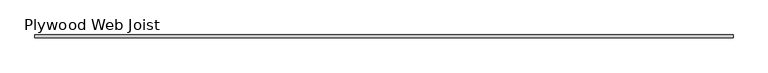
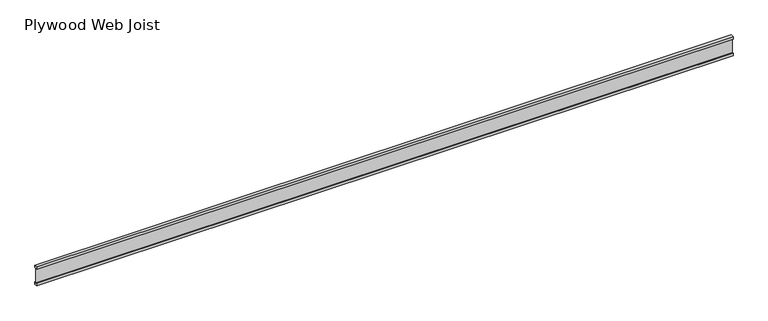
"""IFC4 building model written with IfcOpenShell, lengths in millimetres: beam geometry, Plywood Web Joist : TJI (T.B.D.)."""

from ifc_helpers import new_model, si_unit, frame, origin, place, context, project, spatial, polyline, outline, extrude, source, transform, mapped, element, save


def plywood_web_joist_03ebe8c7(model_context):
    return source(origin(), model_context, "Body", "SweptSolid", [
        extrude(outline(polyline([(-22.225, 150.8125), (22.225, 150.8125), (22.225, 112.7125), (4.7625, 112.7125), (4.7625, 119.0625), (-4.7625, 119.0625), (-4.7625, 112.7125), (-22.225, 112.7125), (-22.225, 150.8125)])), frame((-5185.9151287, 0.0, 0.0), z_axis=(1.0, 0.0, 0.0), x_axis=(0.0, 1.0, 0.0)), (0.0, 0.0, 1.0), 10371.8302575),
        extrude(outline(polyline([(22.225, -112.7125), (22.225, -150.8125), (-22.225, -150.8125), (-22.225, -112.7125), (-4.7625, -112.7125), (-4.7625, -118.3285374), (4.7625, -118.3285374), (4.7625, -112.7125), (22.225, -112.7125)])), frame((-5185.9151287, 0.0, 0.0), z_axis=(1.0, 0.0, 0.0), x_axis=(0.0, 1.0, 0.0)), (0.0, 0.0, 1.0), 10371.8302575),
        extrude(outline(polyline([(5185.9151287, 4.7625), (5185.9151287, -4.7625), (-5185.9151287, -4.7625), (-5185.9151287, 4.7625), (5185.9151287, 4.7625)])), frame((0.0, 0.0, -118.3285374), z_axis=(0.0, 0.0, 1.0), x_axis=(1.0, 0.0, 0.0)), (0.0, 0.0, 1.0), 237.3910374),
    ])


if __name__ == "__main__":
    model = new_model("IFC4")
    model_context = context("Model", 3, world=origin())
    ifc_project = project(units=[si_unit("LENGTHUNIT", "METRE", prefix="MILLI")], contexts=[model_context])
    site = spatial("IfcSite", under=ifc_project)
    building = spatial("IfcBuilding", under=site)
    placement = place(None, origin())
    plywood_web_joist_shape = plywood_web_joist_03ebe8c7(model_context)
    element("IfcBeam", 1, ObjectType="Plywood Web Joist : TJI (T.B.D.)", at=placement, inside=building, context=model_context, shape_type="MappedRepresentation", body=[
        mapped(plywood_web_joist_shape, transform((0.0, 0.0, 0.0), x_axis=(1.0, 0.0, 0.0), y_axis=(0.0, 1.0, 0.0), z_axis=(0.0, 0.0, 1.0))),
    ])
    save(model, "model.ifc")

# Revit data of these elements
# Type "Plywood Web Joist : TJI (T.B.D.)"
#   Assembly Code = "B10"
#   Length [instance default] = 5' - 0"
#   b = 0' - 1 3/4"
#   d = 0' - 11 7/8"
#   Structural Material [instance default] = Softwood, Lumber
# Element 1 (IfcBeam, "Plywood Web Joist : TJI (T.B.D.)")
#   Materials on its faces: "Softwood, Lumber"
# Materials
#   "Softwood, Lumber": class "Wood", colour RGB 144 113 62, transparency 0, Description = "Pinus Echinata", Cost = 0
